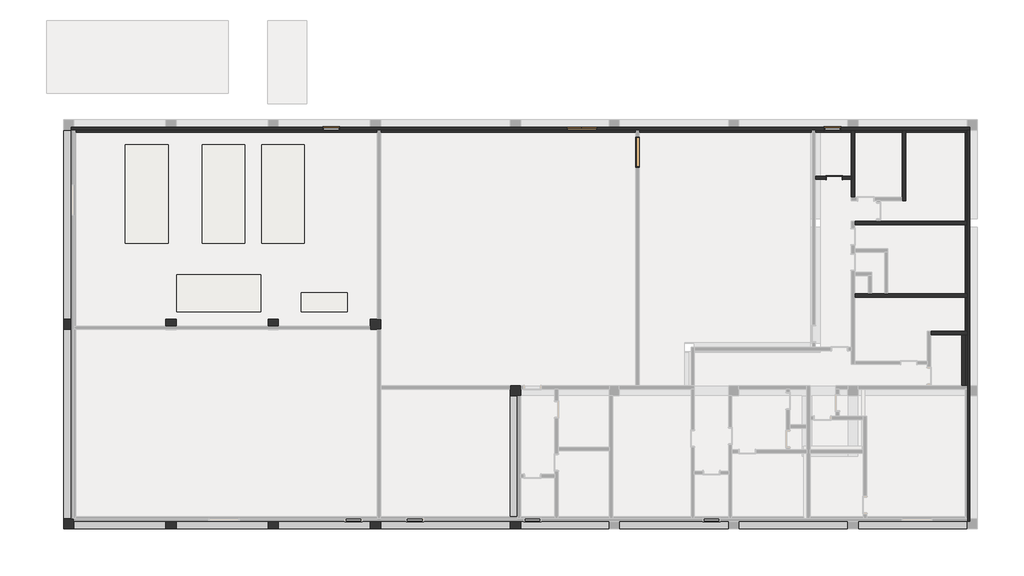
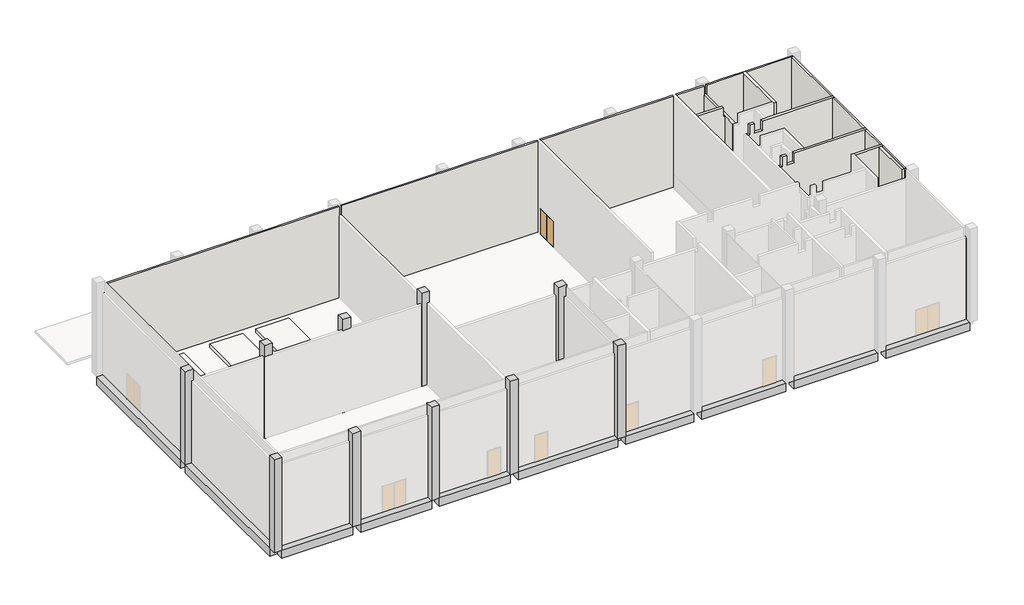
# One storey, part 3 of 4: 19 walls, 10 columns, 5 doors, 5 slabs, 3 beams.
"""IFC4 building model written with IfcOpenShell, lengths in millimetres."""

import ifcopenshell
import ifcopenshell.guid

model = None  # the IFC model being written
_history = None  # IfcOwnerHistory: only IFC2X3 demands one
_inside = {}  # id of a spatial element -> (the spatial element, [elements in it])
_under = {}  # id of a project, library or spatial element -> (it, [spatial elements below it])
_declared = {}  # id of a project -> (the project, [libraries it declares])
_typed = {}  # id of a type object -> (the type object, [elements of that type])
_made_of = {}  # id of a material, layer set ... -> (it, [elements and type objects made of it])


def new_model(schema):
    """Start an empty IFC model of exactly this schema.

    Asked for "IFC4X3", IfcOpenShell would pick the latest addendum, in which some entities
    have other attributes; the version numbers below select the first issue.
    IFC2X3 requires an IfcOwnerHistory on every rooted entity: one is made here for all.
    """
    global model, _history
    if schema == "IFC4X3":
        model = ifcopenshell.file(schema_version=(4, 3, 0, 0))
    else:
        model = ifcopenshell.file(schema=schema)
    _inside.clear()
    _under.clear()
    _declared.clear()
    _typed.clear()
    _made_of.clear()
    _history = None
    if model.schema == "IFC2X3":
        org = make("IfcOrganization", Name="unknown")
        user = make(
            "IfcPersonAndOrganization",
            ThePerson=make("IfcPerson", FamilyName="unknown"),
            TheOrganization=org,
        )
        app = make(
            "IfcApplication",
            ApplicationDeveloper=org,
            Version="unknown",
            ApplicationFullName="unknown",
            ApplicationIdentifier="unknown",
        )
        _history = make(
            "IfcOwnerHistory",
            OwningUser=user,
            OwningApplication=app,
            ChangeAction="ADDED",
            CreationDate=0,
        )
    return model


def make(cls, **values):
    """One entity of the class cls with the attributes given. An attribute that is None is left unset."""
    return model.create_entity(
        cls, **{name: value for name, value in values.items() if value is not None}
    )


def rooted(cls, **values):
    """An entity with a GlobalId (a new one), such as an element, a storey or a relation."""
    return make(cls, GlobalId=ifcopenshell.guid.new(), OwnerHistory=_history, **values)


def si_unit(unit_type, name, prefix=None):
    """IfcSIUnit, for example si_unit("LENGTHUNIT", "METRE", prefix="MILLI")."""
    return make("IfcSIUnit", UnitType=unit_type, Prefix=prefix, Name=name)


def assignment(units):
    """IfcUnitAssignment: the units of a project."""
    return None if units is None else make("IfcUnitAssignment", Units=units)


def point(xyz):
    """IfcCartesianPoint."""
    return None if xyz is None else make("IfcCartesianPoint", Coordinates=xyz)


def direction(xyz):
    """IfcDirection."""
    return None if xyz is None else make("IfcDirection", DirectionRatios=xyz)


def frame(location, z_axis=None, x_axis=None):
    """IfcAxis2Placement3D, a coordinate frame: its origin and axes. An axis left out is left unset."""
    return make(
        "IfcAxis2Placement3D",
        Location=point(location),
        Axis=direction(z_axis),
        RefDirection=direction(x_axis),
    )


def origin():
    """The frame at (0, 0, 0) with its axes left unset."""
    return frame((0.0, 0.0, 0.0))


def origin_with_axes():
    """The frame at (0, 0, 0) with the z axis (0, 0, 1) and the x axis (1, 0, 0) written out."""
    return frame((0.0, 0.0, 0.0), z_axis=(0.0, 0.0, 1.0), x_axis=(1.0, 0.0, 0.0))


def place(relative_to, where):
    """IfcLocalPlacement: puts the frame where relative to a parent placement (None: the world)."""
    return make(
        "IfcLocalPlacement", PlacementRelTo=relative_to, RelativePlacement=where
    )


def context(
    kind, dimensions, precision=None, world=None, true_north=None, identifier=None
):
    """IfcGeometricRepresentationContext, for example the 3D "Model" context."""
    return make(
        "IfcGeometricRepresentationContext",
        ContextIdentifier=identifier,
        ContextType=kind,
        CoordinateSpaceDimension=dimensions,
        Precision=precision,
        WorldCoordinateSystem=world,
        TrueNorth=true_north,
    )


def project(units=None, contexts=None):
    """IfcProject with its units and contexts."""
    return rooted(
        "IfcProject",
        Name="project",
        RepresentationContexts=contexts,
        UnitsInContext=assignment(units),
    )


def spatial(cls, under=None, at=None, **own):
    """A site, building, storey or space (cls), placed at a placement, below another one or the project."""
    s = rooted(cls, ObjectPlacement=at, **own)
    if under is not None:
        _under.setdefault(under.id(), (under, []))[1].append(s)
    return s


def polyline(points):
    """IfcPolyline through the points."""
    return make("IfcPolyline", Points=[point(p) for p in points])


def outline(outer, holes=None, kind="AREA"):
    """IfcArbitraryClosedProfileDef: a profile drawn as a closed curve; with holes, ...WithVoids."""
    if holes is None:
        return make("IfcArbitraryClosedProfileDef", ProfileType=kind, OuterCurve=outer)
    return make(
        "IfcArbitraryProfileDefWithVoids",
        ProfileType=kind,
        OuterCurve=outer,
        InnerCurves=holes,
    )


def extrude(swept, where, along, depth):
    """IfcExtrudedAreaSolid: the profile swept, set in the frame where, extruded along a direction by depth."""
    return make(
        "IfcExtrudedAreaSolid",
        SweptArea=swept,
        Position=where,
        ExtrudedDirection=direction(along),
        Depth=depth,
    )


def faces_of(points, faces, orient=None, outer=None):
    """IfcFace entities. A face is a list of loops; a loop is a list of indices into points, from 0.

    orient and outer hold one flag for each loop. By default every Orientation is true, the
    first loop of a face is its IfcFaceOuterBound and the others are IfcFaceBound.
    """
    made = []
    for i, loops in enumerate(faces):
        bounds = []
        for j, loop in enumerate(loops):
            is_outer = j == 0 if outer is None else outer[i][j]
            bounds.append(
                make(
                    "IfcFaceOuterBound" if is_outer else "IfcFaceBound",
                    Bound=make("IfcPolyLoop", Polygon=[points[k] for k in loop]),
                    Orientation=True if orient is None else orient[i][j],
                )
            )
        made.append(make("IfcFace", Bounds=bounds))
    return made


def faceted_brep(points, faces, orient=None, outer=None, voids=None):
    """IfcFacetedBrep: a solid bounded by flat faces; with voids (closed shells), ...WithVoids."""
    shared = [point(p) for p in points]
    hull = make("IfcClosedShell", CfsFaces=faces_of(shared, faces, orient, outer))
    if voids is None:
        return make("IfcFacetedBrep", Outer=hull)
    return make(
        "IfcFacetedBrepWithVoids",
        Outer=hull,
        Voids=[
            make(cls, CfsFaces=faces_of(shared, fs, o, b)) for cls, fs, o, b in voids
        ],
    )


def shape(context_of_items, identifier, shape_type, items):
    """IfcShapeRepresentation: the items that make up one representation, for example the "Body"."""
    return make(
        "IfcShapeRepresentation",
        ContextOfItems=context_of_items,
        RepresentationIdentifier=identifier,
        RepresentationType=shape_type,
        Items=items,
    )


def source(mapping_origin, context_of_items, identifier, shape_type, items):
    """IfcRepresentationMap: a shape defined once, which mapped items show again and again."""
    return make(
        "IfcRepresentationMap",
        MappingOrigin=mapping_origin,
        MappedRepresentation=shape(context_of_items, identifier, shape_type, items),
    )


def transform(
    local_origin,
    x_axis=None,
    y_axis=None,
    z_axis=None,
    scale=None,
    scale2=None,
    scale3=None,
    uniform=True,
):
    """IfcCartesianTransformationOperator3D, or its non-uniform kind. x_axis, y_axis, z_axis: its Axis1, 2, 3."""
    if uniform:
        return make(
            "IfcCartesianTransformationOperator3D",
            Axis1=direction(x_axis),
            Axis2=direction(y_axis),
            LocalOrigin=point(local_origin),
            Scale=scale,
            Axis3=direction(z_axis),
        )
    return make(
        "IfcCartesianTransformationOperator3DnonUniform",
        Axis1=direction(x_axis),
        Axis2=direction(y_axis),
        LocalOrigin=point(local_origin),
        Scale=scale,
        Axis3=direction(z_axis),
        Scale2=scale2,
        Scale3=scale3,
    )


def mapped(mapping_source, mapping_target):
    """IfcMappedItem: shows the shape of a source again, moved by a transform."""
    return make(
        "IfcMappedItem", MappingSource=mapping_source, MappingTarget=mapping_target
    )


def made_of(thing, what):
    """Note that an element or type object is made of a material, layer set ...; save() writes the relation."""
    if what is not None:
        _made_of.setdefault(what.id(), (what, []))[1].append(thing)
    return thing


def element(
    cls,
    number,
    at=None,
    inside=None,
    cuts=None,
    type_object=None,
    material=None,
    context=None,
    identifier="Body",
    shape_type=None,
    held_by="IfcProductDefinitionShape",
    body=None,
    shapes=None,
    **own,
):
    """One element of the class cls, such as IfcWall. Its Tag is "e" and its number.

    at: its placement. inside: the storey or other place that contains it. cuts: it is an
    opening in that element (IfcRelVoidsElement). A single representation is given by context,
    identifier, shape_type and body (its items); several are given by shapes. held_by: the class
    of the entity that holds the representations. save() writes the other relations.
    """
    e = rooted(cls, Tag="e%d" % number, ObjectPlacement=at, **own)
    if body is not None:
        shapes = [shape(context, identifier, shape_type, body)]
    if shapes is not None:
        e.Representation = make(held_by, Representations=shapes)
    if inside is not None:
        _inside.setdefault(inside.id(), (inside, []))[1].append(e)
    if cuts is not None:
        rooted(
            "IfcRelVoidsElement", RelatingBuildingElement=cuts, RelatedOpeningElement=e
        )
    if type_object is not None:
        _typed.setdefault(type_object.id(), (type_object, []))[1].append(e)
    return made_of(e, material)


def aggregate(whole, parts):
    """IfcRelAggregates: a whole, such as a stair, and the parts it consists of."""
    return rooted("IfcRelAggregates", RelatingObject=whole, RelatedObjects=parts)


def save(model, path):
    """Write the relations noted so far, then the file.

    IfcRelAggregates (storeys below a building ...), IfcRelContainedInSpatialStructure (elements
    in a storey), IfcRelDefinesByType, IfcRelAssociatesMaterial and IfcRelDeclares: one each for
    every whole, place, type object, material and project.
    """
    for whole, parts in _under.values():
        aggregate(whole, parts)
    for where, things in _inside.values():
        rooted(
            "IfcRelContainedInSpatialStructure",
            RelatedElements=things,
            RelatingStructure=where,
        )
    for kind, things in _typed.values():
        rooted("IfcRelDefinesByType", RelatedObjects=things, RelatingType=kind)
    for what, things in _made_of.values():
        rooted("IfcRelAssociatesMaterial", RelatedObjects=things, RelatingMaterial=what)
    for by, libraries in _declared.values():
        rooted("IfcRelDeclares", RelatingContext=by, RelatedDefinitions=libraries)
    model.write(path)


def double_door_steel_580823b0(model_context):
    return source(origin(), model_context, "Body", "SolidModel", [
        extrude(outline(polyline([(880.0, 35.0), (0.0, 35.0), (0.0, 75.0), (880.0, 75.0), (880.0, 35.0)])), frame((0.0, 0.0, 20.0), z_axis=(0.0, 0.0, 1.0), x_axis=(1.0, 0.0, 0.0)), (0.0, 0.0, 1.0), 2060.0),
        extrude(outline(polyline([(0.0, 35.0), (-880.0, 35.0), (-880.0, 75.0), (0.0, 75.0), (0.0, 35.0)])), frame((0.0, 0.0, 20.0), z_axis=(0.0, 0.0, 1.0), x_axis=(1.0, 0.0, 0.0)), (0.0, 0.0, 1.0), 2060.0),
        faceted_brep([(900.0, -75.0, 2100.0), (900.0, 75.0, 2100.0), (-900.0, 75.0, 2100.0), (-900.0, -75.0, 2100.0), (865.0, 35.0, 2065.0), (865.0, -75.0, 2065.0), (-865.0, -75.0, 2065.0), (-865.0, 35.0, 2065.0), (880.0, 75.0, 2080.0), (880.0, 35.0, 2080.0), (-880.0, 35.0, 2080.0), (-880.0, 75.0, 2080.0), (-900.0, 75.0, 0.0), (-900.0, -75.0, 0.0), (-865.0, -75.0, 35.0), (-865.0, 35.0, 35.0), (-880.0, 35.0, 20.0), (-880.0, 75.0, 20.0), (900.0, 75.0, 0.0), (880.0, 75.0, 20.0), (900.0, -75.0, 0.0), (865.0, -75.0, 35.0), (865.0, 35.0, 35.0), (880.0, 35.0, 20.0)], [[[0, 1, 2, 3]], [[4, 5, 6, 7]], [[8, 9, 10, 11]], [[3, 2, 12, 13]], [[7, 6, 14, 15]], [[11, 10, 16, 17]], [[18, 12, 2, 1], [8, 11, 17, 19]], [[13, 12, 18, 20]], [[0, 3, 13, 20], [21, 14, 6, 5]], [[15, 14, 21, 22]], [[23, 16, 10, 9], [4, 7, 15, 22]], [[17, 16, 23, 19]], [[20, 18, 1, 0]], [[22, 21, 5, 4]], [[19, 23, 9, 8]]]),
    ])


def double_door_steel_63a69c0a(model_context):
    return source(origin(), model_context, "Body", "SolidModel", [
        extrude(outline(polyline([(880.0, -60.0), (880.0, -100.0), (0.0, -100.0), (0.0, -60.0), (880.0, -60.0)])), frame((0.0, 0.0, 20.0), z_axis=(0.0, 0.0, 1.0), x_axis=(1.0, 0.0, 0.0)), (0.0, 0.0, 1.0), 2060.0),
        extrude(outline(polyline([(0.0, -60.0), (0.0, -100.0), (-880.0, -100.0), (-880.0, -60.0), (0.0, -60.0)])), frame((0.0, 0.0, 20.0), z_axis=(0.0, 0.0, 1.0), x_axis=(1.0, 0.0, 0.0)), (0.0, 0.0, 1.0), 2060.0),
        faceted_brep([(900.0, 100.0, 2100.0), (-900.0, 100.0, 2100.0), (-900.0, -100.0, 2100.0), (900.0, -100.0, 2100.0), (865.0, -60.0, 2065.0), (-865.0, -60.0, 2065.0), (-865.0, 100.0, 2065.0), (865.0, 100.0, 2065.0), (880.0, -100.0, 2080.0), (-880.0, -100.0, 2080.0), (-880.0, -60.0, 2080.0), (880.0, -60.0, 2080.0), (-900.0, 100.0, 0.0), (-900.0, -100.0, 0.0), (-865.0, -60.0, 35.0), (-865.0, 100.0, 35.0), (-880.0, -100.0, 20.0), (-880.0, -60.0, 20.0), (900.0, -100.0, 0.0), (880.0, -100.0, 20.0), (900.0, 100.0, 0.0), (865.0, 100.0, 35.0), (865.0, -60.0, 35.0), (880.0, -60.0, 20.0)], [[[0, 1, 2, 3]], [[4, 5, 6, 7]], [[8, 9, 10, 11]], [[1, 12, 13, 2]], [[5, 14, 15, 6]], [[9, 16, 17, 10]], [[18, 3, 2, 13], [8, 19, 16, 9]], [[12, 20, 18, 13]], [[0, 20, 12, 1], [21, 7, 6, 15]], [[14, 22, 21, 15]], [[23, 11, 10, 17], [4, 22, 14, 5]], [[16, 19, 23, 17]], [[20, 0, 3, 18]], [[22, 4, 7, 21]], [[19, 8, 11, 23]]]),
    ])


def single_door_steel_b319cbd1(model_context):
    return source(origin(), model_context, "Body", "SolidModel", [
        extrude(outline(polyline([(480.0, -105.0), (-480.0, -105.0), (-480.0, -70.0), (480.0, -70.0), (480.0, -105.0)])), origin_with_axes(), (0.0, 0.0, 1.0), 2130.0),
        faceted_brep([(480.0, -105.0, 0.0), (480.0, -70.0, 0.0), (460.0, -70.0, 0.0), (460.0, 70.0, 0.0), (480.0, 70.0, 0.0), (480.0, 105.0, 0.0), (510.0, 105.0, 0.0), (510.0, -105.0, 0.0), (510.0, -105.0, 2160.0), (-510.0, -105.0, 2160.0), (-510.0, -105.0, 0.0), (-480.0, -105.0, 0.0), (-480.0, -105.0, 2130.0), (480.0, -105.0, 2130.0), (510.0, 105.0, 2160.0), (480.0, 105.0, 2130.0), (-480.0, 105.0, 2130.0), (-480.0, 105.0, 0.0), (-510.0, 105.0, 0.0), (-510.0, 105.0, 2160.0), (480.0, 70.0, 2130.0), (460.0, 70.0, 2110.0), (-460.0, 70.0, 2110.0), (-460.0, 70.0, 0.0), (-480.0, 70.0, 0.0), (-480.0, 70.0, 2130.0), (460.0, -70.0, 2110.0), (480.0, -70.0, 2130.0), (-480.0, -70.0, 2130.0), (-480.0, -70.0, 0.0), (-460.0, -70.0, 0.0), (-460.0, -70.0, 2110.0)], [[[0, 1, 2, 3, 4, 5, 6, 7]], [[7, 8, 9, 10, 11, 12, 13, 0]], [[6, 14, 8, 7]], [[5, 15, 16, 17, 18, 19, 14, 6]], [[4, 20, 15, 5]], [[3, 21, 22, 23, 24, 25, 20, 4]], [[2, 26, 21, 3]], [[1, 27, 28, 29, 30, 31, 26, 2]], [[0, 13, 27, 1]], [[12, 11, 29, 28]], [[11, 10, 18, 17, 24, 23, 30, 29]], [[19, 18, 10, 9]], [[25, 24, 17, 16]], [[31, 30, 23, 22]], [[14, 19, 9, 8]], [[20, 25, 16, 15]], [[26, 31, 22, 21]], [[13, 12, 28, 27]]]),
    ])


def single_door_steel_f73fbc53(model_context):
    return source(origin(), model_context, "Body", "SolidModel", [
        extrude(outline(polyline([(480.0, -130.0), (-480.0, -130.0), (-480.0, -95.0), (480.0, -95.0), (480.0, -130.0)])), origin_with_axes(), (0.0, 0.0, 1.0), 2130.0),
        faceted_brep([(480.0, -130.0, 0.0), (480.0, -95.0, 0.0), (460.0, -95.0, 0.0), (460.0, 95.0, 0.0), (480.0, 95.0, 0.0), (480.0, 130.0, 0.0), (510.0, 130.0, 0.0), (510.0, -130.0, 0.0), (510.0, -130.0, 2160.0), (-510.0, -130.0, 2160.0), (-510.0, -130.0, 0.0), (-480.0, -130.0, 0.0), (-480.0, -130.0, 2130.0), (480.0, -130.0, 2130.0), (510.0, 130.0, 2160.0), (480.0, 130.0, 2130.0), (-480.0, 130.0, 2130.0), (-480.0, 130.0, 0.0), (-510.0, 130.0, 0.0), (-510.0, 130.0, 2160.0), (480.0, 95.0, 2130.0), (460.0, 95.0, 2110.0), (-460.0, 95.0, 2110.0), (-460.0, 95.0, 0.0), (-480.0, 95.0, 0.0), (-480.0, 95.0, 2130.0), (460.0, -95.0, 2110.0), (480.0, -95.0, 2130.0), (-480.0, -95.0, 2130.0), (-480.0, -95.0, 0.0), (-460.0, -95.0, 0.0), (-460.0, -95.0, 2110.0)], [[[0, 1, 2, 3, 4, 5, 6, 7]], [[7, 8, 9, 10, 11, 12, 13, 0]], [[6, 14, 8, 7]], [[5, 15, 16, 17, 18, 19, 14, 6]], [[4, 20, 15, 5]], [[3, 21, 22, 23, 24, 25, 20, 4]], [[2, 26, 21, 3]], [[1, 27, 28, 29, 30, 31, 26, 2]], [[0, 13, 27, 1]], [[12, 11, 29, 28]], [[11, 10, 18, 17, 24, 23, 30, 29]], [[19, 18, 10, 9]], [[25, 24, 17, 16]], [[31, 30, 23, 22]], [[14, 19, 9, 8]], [[20, 25, 16, 15]], [[26, 31, 22, 21]], [[13, 12, 28, 27]]]),
    ])


model = new_model("IFC4")

# Units and contexts
model_context = context("Model", 3, world=origin())
ifc_project = project(units=[si_unit("LENGTHUNIT", "METRE", prefix="MILLI")], contexts=[model_context])

# Site, building, storey
site = spatial("IfcSite", under=ifc_project)
building = spatial("IfcBuilding", under=site)
storey = spatial("IfcBuildingStorey", under=building, Name="TOC(GF)", Elevation=97049.9618634)

# Beams
placement = place(None, origin())
element("IfcBeam", 1, ObjectType="RC Beam_Rectangular : H_SB_AR S16_TG-UG_TG1 600x650", at=placement, inside=storey, context=model_context, shape_type="Brep", body=[
    faceted_brep([(300.0, -19200.0, 97049.9618634), (300.0, -19800.0, 97049.9618634), (5700.0, -19800.0, 97049.9618634), (5700.0, -19200.0, 97049.9618634), (300.0, -19200.0, 96399.9618634), (300.0, -19200.0, 96849.9618634), (5700.0, -19200.0, 96399.9618634), (300.0, -19800.0, 96399.9618634), (5700.0, -19800.0, 96399.9618634)], [[[0, 1, 2, 3]], [[4, 5, 0, 3, 6]], [[7, 4, 6, 8]], [[1, 7, 8, 2]], [[1, 0, 5, 4, 7]], [[3, 2, 8, 6]]]),
    faceted_brep([(26500.0, -19800.0, 97049.9618634), (26500.0, -19200.0, 97049.9618634), (26500.0, -19200.0, 96849.9618634), (26500.0, -19200.0, 96399.9618634), (26500.0, -19800.0, 96399.9618634), (31700.0, -19200.0, 97049.9618634), (31700.0, -19800.0, 97049.9618634), (31700.0, -19800.0, 96399.9618634), (31700.0, -19200.0, 96399.9618634)], [[[0, 1, 2, 3, 4]], [[5, 6, 7, 8]], [[1, 0, 6, 5]], [[3, 2, 1, 5, 8]], [[4, 3, 8, 7]], [[0, 4, 7, 6]]]),
    faceted_brep([(25900.0, -19200.0, 97049.9618634), (25900.0, -19800.0, 97049.9618634), (25900.0, -19800.0, 96399.9618634), (25900.0, -19200.0, 96399.9618634), (25900.0, -19200.0, 96849.9618634), (18300.0, -19800.0, 97049.9618634), (18300.0, -19200.0, 97049.9618634), (18300.0, -19200.0, 96399.9618634), (18300.0, -19800.0, 96399.9618634)], [[[0, 1, 2, 3, 4]], [[5, 6, 7, 8]], [[1, 0, 6, 5]], [[0, 4, 3, 7, 6]], [[3, 2, 8, 7]], [[2, 1, 5, 8]]]),
    faceted_brep([(32300.0, -19800.0, 97049.9618634), (32300.0, -19200.0, 97049.9618634), (32300.0, -19200.0, 96399.9618634), (32300.0, -19800.0, 96399.9618634), (38700.0, -19200.0, 97049.9618634), (38700.0, -19800.0, 97049.9618634), (38700.0, -19800.0, 96399.9618634), (38700.0, -19200.0, 96399.9618634)], [[[0, 1, 2, 3]], [[4, 5, 6, 7]], [[1, 0, 5, 4]], [[2, 1, 4, 7]], [[3, 2, 7, 6]], [[0, 3, 6, 5]]]),
    faceted_brep([(39300.0, -19800.0, 97049.9618634), (39300.0, -19200.0, 97049.9618634), (39300.0, -19200.0, 96399.9618634), (39300.0, -19800.0, 96399.9618634), (45700.0, -19200.0, 97049.9618634), (45700.0, -19800.0, 97049.9618634), (45700.0, -19800.0, 96399.9618634), (45700.0, -19200.0, 96399.9618634)], [[[0, 1, 2, 3]], [[4, 5, 6, 7]], [[1, 0, 5, 4]], [[2, 1, 4, 7]], [[3, 2, 7, 6]], [[0, 3, 6, 5]]]),
    faceted_brep([(46300.0, -19800.0, 97049.9618634), (46300.0, -19200.0, 97049.9618634), (46300.0, -19200.0, 96399.9618634), (46300.0, -19800.0, 96399.9618634), (52700.0, -19200.0, 97049.9618634), (52700.0, -19800.0, 97049.9618634), (52700.0, -19800.0, 96399.9618634), (52700.0, -19200.0, 96399.9618634), (52700.0, -19200.0, 96849.9618634)], [[[0, 1, 2, 3]], [[4, 5, 6, 7, 8]], [[1, 0, 5, 4]], [[2, 1, 4, 8, 7]], [[3, 2, 7, 6]], [[0, 3, 6, 5]]]),
    faceted_brep([(6300.0, -19800.0, 97049.9618634), (6300.0, -19200.0, 97049.9618634), (6300.0, -19200.0, 96399.9618634), (6300.0, -19800.0, 96399.9618634), (11700.0, -19200.0, 97049.9618634), (11700.0, -19800.0, 97049.9618634), (11700.0, -19800.0, 96399.9618634), (11700.0, -19200.0, 96399.9618634)], [[[0, 1, 2, 3]], [[4, 5, 6, 7]], [[1, 0, 5, 4]], [[2, 1, 4, 7]], [[3, 2, 7, 6]], [[0, 3, 6, 5]]]),
    faceted_brep([(12300.0, -19800.0, 97049.9618634), (12300.0, -19200.0, 97049.9618634), (12300.0, -19200.0, 96399.9618634), (12300.0, -19800.0, 96399.9618634), (17700.0, -19200.0, 97049.9618634), (17700.0, -19800.0, 97049.9618634), (17700.0, -19800.0, 96399.9618634), (17700.0, -19200.0, 96399.9618634)], [[[0, 1, 2, 3]], [[4, 5, 6, 7]], [[1, 0, 5, 4]], [[2, 1, 4, 7]], [[3, 2, 7, 6]], [[0, 3, 6, 5]]]),
])
element("IfcBeam", 2, ObjectType="RC Beam_Rectangular : H_SB_AR S16_TG-UG_TG1 600x650", at=placement, inside=storey, context=model_context, shape_type="Brep", body=[
    faceted_brep([(300.0, 3600.0, 97049.9618634), (-300.0, 3600.0, 97049.9618634), (-300.0, -7500.0, 97049.9618634), (300.0, -7500.0, 97049.9618634), (300.0, 3600.0, 96399.9618634), (300.0, 3600.0, 96849.9618634), (300.0, -7500.0, 96399.9618634), (-300.0, 3600.0, 96399.9618634), (-300.0, -7500.0, 96399.9618634)], [[[0, 1, 2, 3]], [[4, 5, 0, 3, 6]], [[7, 4, 6, 8]], [[8, 2, 1, 7]], [[0, 5, 4, 7, 1]], [[3, 2, 8, 6]]]),
    faceted_brep([(300.0, -19200.0, 96399.9618634), (300.0, -19200.0, 96849.9618634), (300.0, -19200.0, 97049.9618634), (-300.0, -19200.0, 97049.9618634), (-300.0, -19200.0, 96399.9618634), (-300.0, -8100.0, 97049.9618634), (300.0, -8100.0, 97049.9618634), (300.0, -8100.0, 96399.9618634), (-300.0, -8100.0, 96399.9618634)], [[[0, 1, 2, 3, 4]], [[5, 6, 7, 8]], [[3, 2, 6, 5]], [[2, 1, 0, 7, 6]], [[0, 4, 8, 7]], [[4, 3, 5, 8]]]),
])
element("IfcBeam", 3, ObjectType="RC Beam_Rectangular : H_SB_AR S16_TG-UG_TG1 600x650", at=placement, inside=storey, context=model_context, shape_type="Brep", body=[
    faceted_brep([(26500.0, -12000.0, 97049.9618634), (25900.0, -12000.0, 97049.9618634), (25900.0, -19200.0, 97049.9618634), (26500.0, -19200.0, 97049.9618634), (25900.0, -12000.0, 96399.9618634), (25900.0, -19200.0, 96399.9618634), (25900.0, -19200.0, 96849.9618634), (26500.0, -12000.0, 96399.9618634), (26500.0, -19200.0, 96399.9618634), (26500.0, -12000.0, 96849.9618634), (26500.0, -19200.0, 96849.9618634)], [[[0, 1, 2, 3]], [[1, 4, 5, 6, 2]], [[4, 7, 8, 5]], [[7, 9, 0, 3, 10, 8]], [[0, 9, 7, 4, 1]], [[3, 2, 6, 5, 8, 10]]]),
])

# Columns
element("IfcColumn", 4, ObjectType="RC_Column_Rectangular : H_SC_AR S15_RC Col-AG_C1 600x600", at=placement, inside=storey, context=model_context, shape_type="Brep", body=[
    faceted_brep([(300.0, -19200.0, 97049.9618634), (300.0, -19350.0, 97049.9618634), (300.0, -19800.0, 97049.9618634), (-300.0, -19800.0, 97049.9618634), (-300.0, -19200.0, 97049.9618634), (300.0, -19200.0, 104550.0), (300.0, -19800.0, 104550.0), (300.0, -19200.0, 103650.0), (-300.0, -19800.0, 104550.0), (-300.0, -19200.0, 104550.0)], [[[0, 1, 2, 3, 4]], [[5, 6, 2, 1, 0, 7]], [[6, 8, 3, 2]], [[8, 9, 4, 3]], [[9, 5, 7, 0, 4]], [[5, 9, 8, 6]]]),
])
element("IfcColumn", 5, ObjectType="RC_Column_Rectangular : H_SC_AR S15_RC Col-AG_C1 600x600", at=placement, inside=storey, context=model_context, shape_type="Brep", body=[
    faceted_brep([(300.0, -7500.0, 97049.9618634), (300.0, -8100.0, 97049.9618634), (-300.0, -8100.0, 97049.9618634), (-300.0, -7500.0, 97049.9618634), (300.0, -7500.0, 104550.0), (300.0, -8100.0, 104550.0), (300.0, -8100.0, 103650.0), (300.0, -7500.0, 103650.0), (-300.0, -8100.0, 104550.0), (-300.0, -8100.0, 103650.0), (-300.0, -7500.0, 104550.0), (-300.0, -7500.0, 103650.0)], [[[0, 1, 2, 3]], [[4, 5, 6, 1, 0, 7]], [[5, 8, 9, 2, 1, 6]], [[8, 10, 11, 3, 2, 9]], [[10, 4, 7, 0, 3, 11]], [[4, 10, 8, 5]]]),
])
element("IfcColumn", 6, ObjectType="RC_Column_Rectangular : H_SC_AR S15_RC Col-AG_C1 600x600", at=placement, inside=storey, context=model_context, shape_type="Brep", body=[
    faceted_brep([(26500.0, -19200.0, 97049.9618634), (26500.0, -19800.0, 97049.9618634), (25900.0, -19800.0, 97049.9618634), (25900.0, -19200.0, 97049.9618634), (26500.0, -19200.0, 104550.0), (26500.0, -19800.0, 104550.0), (26500.0, -19800.0, 103650.0), (26500.0, -19200.0, 103650.0), (25900.0, -19800.0, 104550.0), (25900.0, -19800.0, 103650.0), (25900.0, -19200.0, 104550.0), (25900.0, -19200.0, 103650.0), (25950.0, -19200.0, 104550.0), (26450.0, -19200.0, 104550.0)], [[[0, 1, 2, 3]], [[4, 5, 6, 1, 0, 7]], [[5, 8, 9, 2, 1, 6]], [[8, 10, 11, 3, 2, 9]], [[10, 12, 13, 4, 7, 0, 3, 11]], [[4, 13, 12, 10, 8, 5]]]),
])
element("IfcColumn", 7, ObjectType="RC_Column_Rectangular : H_SC_AR S15_RC Col-AG_C1 600x600", at=placement, inside=storey, context=model_context, shape_type="Brep", body=[
    faceted_brep([(6300.0, -19200.0, 97049.9618634), (6300.0, -19800.0, 97049.9618634), (5700.0, -19800.0, 97049.9618634), (5700.0, -19200.0, 97049.9618634), (6300.0, -19200.0, 104550.0), (6300.0, -19800.0, 104550.0), (6300.0, -19800.0, 103650.0), (6300.0, -19200.0, 103650.0), (5700.0, -19800.0, 104550.0), (5700.0, -19800.0, 103650.0), (5700.0, -19200.0, 104550.0), (5700.0, -19200.0, 103650.0), (5800.0, -19200.0, 104550.0), (6200.0, -19200.0, 104550.0)], [[[0, 1, 2, 3]], [[4, 5, 6, 1, 0, 7]], [[5, 8, 9, 2, 1, 6]], [[8, 10, 11, 3, 2, 9]], [[10, 12, 13, 4, 7, 0, 3, 11]], [[4, 13, 12, 10, 8, 5]]]),
])
element("IfcColumn", 8, ObjectType="RC_Column_Rectangular : H_SC_AR S15_RC Col-AG_C1 600x600", at=placement, inside=storey, context=model_context, shape_type="Brep", body=[
    faceted_brep([(6300.0, -7500.0, 97049.9618634), (6300.0, -8100.0, 97049.9618634), (5700.0, -8100.0, 97049.9618634), (5700.0, -7500.0, 97049.9618634), (6300.0, -7500.0, 104550.0), (6300.0, -8100.0, 104550.0), (6300.0, -8100.0, 103650.0), (6300.0, -7500.0, 103650.0), (6200.0, -8100.0, 104550.0), (5800.0, -8100.0, 104550.0), (5700.0, -8100.0, 104550.0), (5700.0, -8100.0, 103650.0), (5700.0, -7500.0, 104550.0), (5700.0, -7500.0, 103650.0), (5800.0, -7500.0, 104550.0), (6200.0, -7500.0, 104550.0)], [[[0, 1, 2, 3]], [[4, 5, 6, 1, 0, 7]], [[5, 8, 9, 10, 11, 2, 1, 6]], [[10, 12, 13, 3, 2, 11]], [[12, 14, 15, 4, 7, 0, 3, 13]], [[4, 15, 14, 12, 10, 9, 8, 5]]]),
])
element("IfcColumn", 9, ObjectType="RC_Column_Rectangular : H_SC_AR S15_RC Col-AG_C1 600x600", at=placement, inside=storey, context=model_context, shape_type="Brep", body=[
    faceted_brep([(12300.0, -19200.0, 97049.9618634), (12300.0, -19800.0, 97049.9618634), (11700.0, -19800.0, 97049.9618634), (11700.0, -19200.0, 97049.9618634), (12300.0, -19200.0, 104550.0), (12300.0, -19800.0, 104550.0), (12300.0, -19800.0, 103650.0), (12300.0, -19200.0, 103650.0), (11700.0, -19800.0, 104550.0), (11700.0, -19800.0, 103650.0), (11700.0, -19200.0, 104550.0), (11700.0, -19200.0, 103650.0), (11800.0, -19200.0, 104550.0), (12200.0, -19200.0, 104550.0)], [[[0, 1, 2, 3]], [[4, 5, 6, 1, 0, 7]], [[5, 8, 9, 2, 1, 6]], [[8, 10, 11, 3, 2, 9]], [[10, 12, 13, 4, 7, 0, 3, 11]], [[4, 13, 12, 10, 8, 5]]]),
])
element("IfcColumn", 10, ObjectType="RC_Column_Rectangular : H_SC_AR S15_RC Col-AG_C1 600x600", at=placement, inside=storey, context=model_context, shape_type="Brep", body=[
    faceted_brep([(12300.0, -7500.0, 97049.9618634), (12300.0, -8100.0, 97049.9618634), (11700.0, -8100.0, 97049.9618634), (11700.0, -7500.0, 97049.9618634), (12300.0, -7500.0, 104550.0), (12300.0, -8100.0, 104550.0), (12300.0, -8100.0, 103650.0), (12300.0, -7500.0, 103650.0), (12200.0, -8100.0, 104550.0), (11800.0, -8100.0, 104550.0), (11700.0, -8100.0, 104550.0), (11700.0, -8100.0, 103650.0), (11700.0, -7500.0, 104550.0), (11700.0, -7500.0, 103650.0), (11800.0, -7500.0, 104550.0), (12200.0, -7500.0, 104550.0)], [[[0, 1, 2, 3]], [[4, 5, 6, 1, 0, 7]], [[5, 8, 9, 10, 11, 2, 1, 6]], [[10, 12, 13, 3, 2, 11]], [[12, 14, 15, 4, 7, 0, 3, 13]], [[4, 15, 14, 12, 10, 9, 8, 5]]]),
])
element("IfcColumn", 11, ObjectType="RC_Column_Rectangular : H_SC_AR S15_RC Col-AG_C1 600x600", at=placement, inside=storey, context=model_context, shape_type="Brep", body=[
    faceted_brep([(18300.0, -19200.0, 97049.9618634), (18300.0, -19800.0, 97049.9618634), (17700.0, -19800.0, 97049.9618634), (17700.0, -19200.0, 97049.9618634), (18300.0, -19200.0, 104550.0), (18300.0, -19800.0, 104550.0), (18300.0, -19800.0, 103650.0), (18300.0, -19200.0, 103650.0), (17700.0, -19800.0, 104550.0), (17700.0, -19800.0, 103650.0), (17700.0, -19200.0, 104550.0), (17700.0, -19200.0, 103650.0)], [[[0, 1, 2, 3]], [[4, 5, 6, 1, 0, 7]], [[5, 8, 9, 2, 1, 6]], [[8, 10, 11, 3, 2, 9]], [[10, 4, 7, 0, 3, 11]], [[4, 10, 8, 5]]]),
])
element("IfcColumn", 12, ObjectType="RC_Column_Rectangular : H_SC_AR S15_RC Col-AG_C1 600x600", at=placement, inside=storey, context=model_context, shape_type="Brep", body=[
    faceted_brep([(18300.0, -7500.0, 97049.9618634), (18300.0, -8100.0, 97049.9618634), (17700.0, -8100.0, 97049.9618634), (17700.0, -7500.0, 97049.9618634), (18300.0, -7500.0, 104550.0), (18300.0, -8100.0, 104550.0), (18300.0, -8100.0, 103650.0), (18300.0, -7500.0, 103650.0), (17700.0, -8100.0, 104550.0), (17700.0, -8100.0, 103650.0), (17700.0, -7500.0, 104550.0), (17700.0, -7500.0, 103650.0)], [[[0, 1, 2, 3]], [[4, 5, 6, 1, 0, 7]], [[5, 8, 9, 2, 1, 6]], [[8, 10, 11, 3, 2, 9]], [[10, 4, 7, 0, 3, 11]], [[4, 10, 8, 5]]]),
])
element("IfcColumn", 13, ObjectType="RC_Column_Rectangular : H_SC_AR S15_RC Col-AG_C2 600x600 2", at=placement, inside=storey, context=model_context, shape_type="SweptSolid", body=[
    extrude(outline(polyline([(26500.0, -11400.0), (26500.0, -12000.0), (25900.0, -12000.0), (25900.0, -11400.0), (26500.0, -11400.0)])), frame((0.0, 0.0, 97049.9618634), z_axis=(0.0, 0.0, 1.0), x_axis=(1.0, 0.0, 0.0)), (0.0, 0.0, 1.0), 7500.0381366),
])

# Doors
double_door_steel_shape = double_door_steel_580823b0(model_context)
element("IfcDoor", 14, ObjectType="Double Door_Steel : H_DR_AR B12_Door_Double FSD 02", at=placement, inside=storey, context=model_context, shape_type="MappedRepresentation", body=[
    mapped(double_door_steel_shape, transform((30100.0, 3675.0, 97049.9618634), x_axis=(1.0, 0.0, 0.0), y_axis=(0.0, 1.0, 0.0), z_axis=(0.0, 0.0, 1.0))),
])
double_door_steel_2_shape = double_door_steel_63a69c0a(model_context)
element("IfcDoor", 15, ObjectType="Double Door_Steel : H_DR_AR B12_Door_Double FSD 02", at=placement, inside=storey, context=model_context, shape_type="MappedRepresentation", body=[
    mapped(double_door_steel_2_shape, transform((33350.0, 2300.0, 97049.9618634), x_axis=(0.0, -1.0, 0.0), y_axis=(1.0, 0.0, 0.0), z_axis=(0.0, 0.0, 1.0))),
])
single_door_steel_shape = single_door_steel_b319cbd1(model_context)
element("IfcDoor", 16, ObjectType="Single Door_Steel : H_DR_AR B12_Door_Single FSD 01", at=placement, inside=storey, context=model_context, shape_type="MappedRepresentation", body=[
    mapped(single_door_steel_shape, transform((44800.0, 3675.0, 97049.9618634), x_axis=(-1.0, 0.0, 0.0), y_axis=(0.0, -1.0, 0.0), z_axis=(0.0, 0.0, 1.0))),
])
element("IfcDoor", 17, ObjectType="Single Door_Steel : H_DR_AR B12_Door_Single FSD 01", at=placement, inside=storey, context=model_context, shape_type="MappedRepresentation", body=[
    mapped(single_door_steel_shape, transform((15400.0, 3675.0, 97049.9618634), x_axis=(-1.0, 0.0, 0.0), y_axis=(0.0, -1.0, 0.0), z_axis=(0.0, 0.0, 1.0))),
])
single_door_steel_2_shape = single_door_steel_f73fbc53(model_context)
element("IfcDoor", 18, ObjectType="Single Door_Steel : H_DR_AR B12_Door_Single FSD 01", at=placement, inside=storey, context=model_context, shape_type="MappedRepresentation", body=[
    mapped(single_door_steel_2_shape, transform((44900.0, 800.0, 97049.9618634), x_axis=(-1.0, 0.0, 0.0), y_axis=(0.0, -1.0, 0.0), z_axis=(0.0, 0.0, 1.0))),
])

# Slabs
element("IfcSlab", 19, ObjectType="H_SF_AR B01_EQ Fdn_EF3 2500x5800x300", at=placement, inside=storey, context=model_context, shape_type="SweptSolid", body=[
    extrude(outline(polyline([(5825.0, 2750.0), (5825.0, -3050.0), (3325.0, -3050.0), (3325.0, 2750.0), (5825.0, 2750.0)])), frame((0.0, 0.0, 97049.9618634), z_axis=(0.0, 0.0, 1.0), x_axis=(1.0, 0.0, 0.0)), (0.0, 0.0, 1.0), 300.0),
])
element("IfcSlab", 20, ObjectType="H_SF_AR B01_EQ Fdn_EF3 2500x5800x300", at=placement, inside=storey, context=model_context, shape_type="SweptSolid", body=[
    extrude(outline(polyline([(10325.0, 2750.0), (10325.0, -3050.0), (7825.0, -3050.0), (7825.0, 2750.0), (10325.0, 2750.0)])), frame((0.0, 0.0, 97049.9618634), z_axis=(0.0, 0.0, 1.0), x_axis=(1.0, 0.0, 0.0)), (0.0, 0.0, 1.0), 300.0),
])
element("IfcSlab", 21, ObjectType="H_SF_AR B01_EQ Fdn_EF3 2500x5800x300", at=placement, inside=storey, context=model_context, shape_type="SweptSolid", body=[
    extrude(outline(polyline([(13825.0, 2750.0), (13825.0, -3050.0), (11325.0, -3050.0), (11325.0, 2750.0), (13825.0, 2750.0)])), frame((0.0, 0.0, 97049.9618634), z_axis=(0.0, 0.0, 1.0), x_axis=(1.0, 0.0, 0.0)), (0.0, 0.0, 1.0), 300.0),
])
element("IfcSlab", 22, ObjectType="H_SF_AR B01_EQ Fdn_EF4 4900x2300x200", at=placement, inside=storey, context=model_context, shape_type="SweptSolid", body=[
    extrude(outline(polyline([(11250.0, -4886.2922312), (11250.0, -7050.0), (6350.0, -7050.0), (6350.0, -4886.2922312), (11250.0, -4886.2922312)])), frame((0.0, 0.0, 97049.9618634), z_axis=(0.0, 0.0, 1.0), x_axis=(1.0, 0.0, 0.0)), (0.0, 0.0, 1.0), 200.0),
])
element("IfcSlab", 23, ObjectType="H_SF_AR B01_EQ Fdn_EF5 2700x1100x200", at=placement, inside=storey, context=model_context, shape_type="SweptSolid", body=[
    extrude(outline(polyline([(16350.0, -5950.0), (16350.0, -7050.0), (13650.0, -7050.0), (13650.0, -5950.0), (16350.0, -5950.0)])), frame((0.0, 0.0, 97049.9618634), z_axis=(0.0, 0.0, 1.0), x_axis=(1.0, 0.0, 0.0)), (0.0, 0.0, 1.0), 200.0),
])

# Walls
element("IfcWall", 24, ObjectType="H_WA_AR B02_Ext Wall RC-AG_EW5", at=placement, inside=storey, context=model_context, shape_type="Brep", body=[
    faceted_brep([(44290.0, 3600.0, 97049.9618634), (44290.0, 3600.0, 99209.9618634), (45310.0, 3600.0, 99209.9618634), (45310.0, 3600.0, 97049.9618634), (45900.0, 3600.0, 97049.9618634), (46100.0, 3600.0, 97049.9618634), (48900.0, 3600.0, 97049.9618634), (49100.0, 3600.0, 97049.9618634), (52700.0, 3600.0, 97049.9618634), (52850.0, 3600.0, 97049.9618634), (52850.0, 3600.0, 103650.0), (52700.0, 3600.0, 103650.0), (46300.0, 3600.0, 103650.0), (46100.0, 3600.0, 103650.0), (45900.0, 3600.0, 103650.0), (45700.0, 3600.0, 103650.0), (39300.0, 3600.0, 103650.0), (38700.0, 3600.0, 103650.0), (32300.0, 3600.0, 103650.0), (31700.0, 3600.0, 103650.0), (26500.0, 3600.0, 103650.0), (25900.0, 3600.0, 103650.0), (18300.0, 3600.0, 103650.0), (18100.0, 3600.0, 103650.0), (17700.0, 3600.0, 103650.0), (12300.0, 3600.0, 103650.0), (11700.0, 3600.0, 103650.0), (6300.0, 3600.0, 103650.0), (5700.0, 3600.0, 103650.0), (300.0, 3600.0, 103650.0), (150.0, 3600.0, 103650.0), (150.0, 3600.0, 97049.9618634), (300.0, 3600.0, 97049.9618634), (426.0, 3600.0, 97049.9618634), (14890.0, 3600.0, 97049.9618634), (14890.0, 3600.0, 99209.9618634), (15910.0, 3600.0, 99209.9618634), (15910.0, 3600.0, 97049.9618634), (18100.0, 3600.0, 97049.9618634), (18300.0, 3600.0, 97049.9618634), (29200.0, 3600.0, 97049.9618634), (29200.0, 3600.0, 99149.9618634), (31000.0, 3600.0, 99149.9618634), (31000.0, 3600.0, 97049.9618634), (33250.0, 3600.0, 97049.9618634), (33450.0, 3600.0, 97049.9618634), (43600.0, 3600.0, 97049.9618634), (43800.0, 3600.0, 97049.9618634), (150.0, 3750.0, 103650.0), (52850.0, 3750.0, 103650.0), (52850.0, 3750.0, 97049.9618634), (45310.0, 3750.0, 97049.9618634), (45310.0, 3750.0, 99209.9618634), (44290.0, 3750.0, 99209.9618634), (44290.0, 3750.0, 97049.9618634), (31000.0, 3750.0, 97049.9618634), (31000.0, 3750.0, 99149.9618634), (29200.0, 3750.0, 99149.9618634), (29200.0, 3750.0, 97049.9618634), (15910.0, 3750.0, 97049.9618634), (15910.0, 3750.0, 99209.9618634), (14890.0, 3750.0, 99209.9618634), (14890.0, 3750.0, 97049.9618634), (150.0, 3750.0, 97049.9618634)], [[[0, 1, 2, 3, 4, 5, 6, 7, 8, 9, 10, 11, 12, 13, 14, 15, 16, 17, 18, 19, 20, 21, 22, 23, 24, 25, 26, 27, 28, 29, 30, 31, 32, 33, 34, 35, 36, 37, 38, 39, 40, 41, 42, 43, 44, 45, 46, 47]], [[48, 49, 50, 51, 52, 53, 54, 55, 56, 57, 58, 59, 60, 61, 62, 63]], [[50, 9, 8, 7, 6, 5, 4, 3, 51]], [[31, 63, 62, 34, 33, 32]], [[54, 0, 47, 46, 45, 44, 43, 55]], [[58, 40, 39, 38, 37, 59]], [[9, 50, 49, 10]], [[63, 31, 30, 48]], [[48, 30, 29, 28, 27, 26, 25, 24, 23, 22, 21, 20, 19, 18, 17, 16, 15, 14, 13, 12, 11, 10, 49]], [[1, 0, 54, 53]], [[2, 1, 53, 52]], [[3, 2, 52, 51]], [[42, 56, 55, 43]], [[56, 42, 41, 57]], [[57, 41, 40, 58]], [[35, 34, 62, 61]], [[36, 35, 61, 60]], [[37, 36, 60, 59]]]),
])
element("IfcWall", 25, ObjectType="H_WA_AR B02_Ext Wall RC-AG_EW5", at=placement, inside=storey, context=model_context, shape_type="Brep", body=[
    faceted_brep([(52700.0, 3600.0, 97049.9618634), (52700.0, 3474.0, 97049.9618634), (52700.0, -1750.0, 97049.9618634), (52700.0, -1950.0, 97049.9618634), (52700.0, -6015.0, 97049.9618634), (52700.0, -6215.0, 97049.9618634), (52700.0, -8200.0, 97049.9618634), (52700.0, -8400.0, 97049.9618634), (52700.0, -11400.0, 97049.9618634), (52700.0, -11600.0, 97049.9618634), (52700.0, -19200.0, 97049.9618634), (52700.0, -19350.0, 97049.9618634), (52700.0, -19350.0, 103650.0), (52700.0, -19200.0, 103650.0), (52700.0, -12000.0, 103650.0), (52700.0, -11600.0, 103650.0), (52700.0, -11400.0, 103650.0), (52700.0, 3600.0, 103650.0), (52850.0, -19350.0, 97049.9618634), (52850.0, 3600.0, 97049.9618634), (52850.0, 3600.0, 103650.0), (52850.0, -19350.0, 103650.0)], [[[0, 1, 2, 3, 4, 5, 6, 7, 8, 9, 10, 11, 12, 13, 14, 15, 16, 17]], [[18, 19, 20, 21]], [[11, 10, 9, 8, 7, 6, 5, 4, 3, 2, 1, 0, 19, 18]], [[19, 0, 17, 20]], [[11, 18, 21, 12]], [[12, 21, 20, 17, 16, 15, 14, 13]]]),
])
element("IfcWall", 26, ObjectType="H_WA_AR B02_Int Wall MA_IW1 T200", at=placement, inside=storey, context=model_context, shape_type="SweptSolid", body=[
    extrude(outline(polyline([(104400.0, 43800.0), (97049.9618634, 43800.0), (97049.9618634, 44390.0), (99209.9618634, 44390.0), (99209.9618634, 45410.0), (97049.9618634, 45410.0), (97049.9618634, 45900.0), (103650.0, 45900.0), (103650.0, 45750.0), (104400.0, 45750.0), (104400.0, 43800.0)])), frame((0.0, 700.0, 0.0), z_axis=(0.0, 1.0, 0.0), x_axis=(0.0, 0.0, 1.0)), (0.0, 0.0, 1.0), 200.0),
])
element("IfcWall", 27, ObjectType="H_WA_AR B02_Int Wall MA_IW1 T200", at=placement, inside=storey, context=model_context, shape_type="Brep", body=[
    faceted_brep([(48900.0, 3600.0, 97049.9618634), (48900.0, 3474.0, 97049.9618634), (48900.0, -350.0, 97049.9618634), (48900.0, -550.0, 97049.9618634), (48900.0, -550.0, 104400.0), (48900.0, -350.0, 104400.0), (48900.0, 3600.0, 104400.0), (49100.0, -550.0, 97049.9618634), (49100.0, 3474.0, 97049.9618634), (49100.0, 3600.0, 97049.9618634), (49100.0, 3600.0, 104400.0), (49100.0, -550.0, 104400.0)], [[[0, 1, 2, 3, 4, 5, 6]], [[7, 8, 9, 10, 11]], [[3, 2, 1, 0, 9, 8, 7]], [[9, 0, 6, 10]], [[3, 7, 11, 4]], [[6, 5, 4, 11, 10]]]),
])
element("IfcWall", 28, ObjectType="H_WA_AR B02_Int Wall MA_IW1 T200", at=placement, inside=storey, context=model_context, shape_type="Brep", body=[
    faceted_brep([(52700.0, -1750.0, 97049.9618634), (52574.0, -1750.0, 97049.9618634), (47600.0, -1750.0, 97049.9618634), (47400.0, -1750.0, 97049.9618634), (46100.0, -1750.0, 97049.9618634), (46100.0, -1750.0, 103650.0), (46250.0, -1750.0, 103650.0), (46250.0, -1750.0, 104400.0), (46600.0, -1750.0, 104400.0), (46600.0, -1750.0, 103650.0), (47200.0, -1750.0, 103650.0), (47200.0, -1750.0, 104400.0), (47400.0, -1750.0, 104400.0), (47600.0, -1750.0, 104400.0), (52700.0, -1750.0, 104400.0), (46100.0, -1950.0, 97049.9618634), (52574.0, -1950.0, 97049.9618634), (52700.0, -1950.0, 97049.9618634), (52700.0, -1950.0, 104400.0), (47200.0, -1950.0, 104400.0), (47200.0, -1950.0, 103650.0), (46600.0, -1950.0, 103650.0), (46600.0, -1950.0, 104400.0), (46250.0, -1950.0, 104400.0), (46250.0, -1950.0, 103650.0), (46100.0, -1950.0, 103650.0)], [[[0, 1, 2, 3, 4, 5, 6, 7, 8, 9, 10, 11, 12, 13, 14]], [[15, 16, 17, 18, 19, 20, 21, 22, 23, 24, 25]], [[4, 3, 2, 1, 0, 17, 16, 15]], [[17, 0, 14, 18]], [[7, 23, 22, 8]], [[18, 14, 13, 12, 11, 19]], [[24, 6, 5, 25]], [[6, 24, 23, 7]], [[21, 9, 8, 22]], [[9, 21, 20, 10]], [[10, 20, 19, 11]], [[4, 15, 25, 5]]]),
])
element("IfcWall", 29, ObjectType="H_WA_AR B02_Int Wall MA_IW1 T200", at=placement, inside=storey, context=model_context, shape_type="Brep", body=[
    faceted_brep([(52700.0, -6015.0, 97049.9618634), (52574.0, -6015.0, 97049.9618634), (48050.0, -6015.0, 97049.9618634), (47850.0, -6015.0, 97049.9618634), (47100.0, -6015.0, 97049.9618634), (46900.0, -6015.0, 97049.9618634), (46100.0, -6015.0, 97049.9618634), (46100.0, -6015.0, 103650.0), (46250.0, -6015.0, 103650.0), (46250.0, -6015.0, 104400.0), (46600.0, -6015.0, 104400.0), (46600.0, -6015.0, 103650.0), (47200.0, -6015.0, 103650.0), (47200.0, -6015.0, 104400.0), (47850.0, -6015.0, 104400.0), (48050.0, -6015.0, 104400.0), (52700.0, -6015.0, 104400.0), (46100.0, -6215.0, 97049.9618634), (52574.0, -6215.0, 97049.9618634), (52700.0, -6215.0, 97049.9618634), (52700.0, -6215.0, 104400.0), (47200.0, -6215.0, 104400.0), (47200.0, -6215.0, 103650.0), (46600.0, -6215.0, 103650.0), (46600.0, -6215.0, 104400.0), (46250.0, -6215.0, 104400.0), (46250.0, -6215.0, 103650.0), (46100.0, -6215.0, 103650.0)], [[[0, 1, 2, 3, 4, 5, 6, 7, 8, 9, 10, 11, 12, 13, 14, 15, 16]], [[17, 18, 19, 20, 21, 22, 23, 24, 25, 26, 27]], [[6, 5, 4, 3, 2, 1, 0, 19, 18, 17]], [[6, 17, 27, 7]], [[19, 0, 16, 20]], [[9, 25, 24, 10]], [[20, 16, 15, 14, 13, 21]], [[26, 8, 7, 27]], [[8, 26, 25, 9]], [[23, 11, 10, 24]], [[11, 23, 22, 12]], [[12, 22, 21, 13]]]),
])
element("IfcWall", 30, ObjectType="H_WA_AR B02_Int Wall MA_IW1 T200", at=placement, inside=storey, context=model_context, shape_type="SweptSolid", body=[
    extrude(outline(polyline([(52574.0, -8400.0), (52574.0, -11400.0), (52374.0, -11400.0), (52374.0, -8400.0), (52574.0, -8400.0)])), frame((0.0, 0.0, 97049.9618634), z_axis=(0.0, 0.0, 1.0), x_axis=(1.0, 0.0, 0.0)), (0.0, 0.0, 1.0), 7350.0381366),
])
element("IfcWall", 31, ObjectType="H_WA_AR B02_Int Wall MA_IW1 T200", at=placement, inside=storey, context=model_context, shape_type="Brep", body=[
    faceted_brep([(50570.0, -8400.0, 97049.9618634), (52374.0, -8400.0, 97049.9618634), (52574.0, -8400.0, 97049.9618634), (52700.0, -8400.0, 97049.9618634), (52700.0, -8400.0, 104400.0), (52574.0, -8400.0, 104400.0), (52374.0, -8400.0, 104400.0), (50570.0, -8400.0, 104400.0), (52700.0, -8200.0, 97049.9618634), (52574.0, -8200.0, 97049.9618634), (50570.0, -8200.0, 97049.9618634), (50570.0, -8200.0, 104400.0), (52700.0, -8200.0, 104400.0)], [[[0, 1, 2, 3, 4, 5, 6, 7]], [[8, 9, 10, 11, 12]], [[3, 2, 1, 0, 10, 9, 8]], [[10, 0, 7, 11]], [[3, 8, 12, 4]], [[7, 6, 5, 4, 12, 11]]]),
])
element("IfcWall", 32, ObjectType="H_WA_AR B02_Int Wall MA_IW1 T200", at=placement, inside=storey, context=model_context, shape_type="Brep", body=[
    faceted_brep([(46100.0, -350.0, 97049.9618634), (46100.0, 3474.0, 97049.9618634), (46100.0, 3600.0, 97049.9618634), (46100.0, 3600.0, 103650.0), (46100.0, -350.0, 103650.0), (45900.0, 3600.0, 97049.9618634), (45900.0, 3474.0, 97049.9618634), (45900.0, 900.0, 97049.9618634), (45900.0, 700.0, 97049.9618634), (45900.0, -350.0, 97049.9618634), (45900.0, -350.0, 103650.0), (45900.0, 700.0, 103650.0), (45900.0, 900.0, 103650.0), (45900.0, 3600.0, 103650.0)], [[[0, 1, 2, 3, 4]], [[5, 6, 7, 8, 9, 10, 11, 12, 13]], [[2, 1, 0, 9, 8, 7, 6, 5]], [[2, 5, 13, 3]], [[4, 3, 13, 12, 11, 10]], [[9, 0, 4, 10]]]),
])
element("IfcWall", 33, ObjectType="H_WA_AR B02_Ext Wall DY-IN_EW1_VB", at=placement, inside=storey, context=model_context, shape_type="Brep", body=[
    faceted_brep([(426.0, 3474.0, 97049.9618634), (18100.0, 3474.0, 97049.9618634), (18100.0, 3474.0, 104400.0), (426.0, 3474.0, 104400.0), (18100.0, 3600.0, 97049.9618634), (426.0, 3600.0, 97049.9618634), (426.0, 3600.0, 104400.0), (2800.0, 3600.0, 104400.0), (3200.0, 3600.0, 104400.0), (5800.0, 3600.0, 104400.0), (6200.0, 3600.0, 104400.0), (8800.0, 3600.0, 104400.0), (9200.0, 3600.0, 104400.0), (11800.0, 3600.0, 104400.0), (12200.0, 3600.0, 104400.0), (14800.0, 3600.0, 104400.0), (15200.0, 3600.0, 104400.0), (17700.0, 3600.0, 104400.0), (18100.0, 3600.0, 104400.0), (18100.0, 3600.0, 103650.0)], [[[0, 1, 2, 3]], [[4, 5, 6, 7, 8, 9, 10, 11, 12, 13, 14, 15, 16, 17, 18, 19]], [[1, 0, 5, 4]], [[1, 4, 19, 18, 2]], [[5, 0, 3, 6]], [[3, 2, 18, 17, 16, 15, 14, 13, 12, 11, 10, 9, 8, 7, 6]]]),
])
element("IfcWall", 34, ObjectType="H_WA_AR B02_Ext Wall DY-IN_EW1_VB", at=placement, inside=storey, context=model_context, shape_type="Brep", body=[
    faceted_brep([(18300.0, 3474.0, 97049.9618634), (33250.0, 3474.0, 97049.9618634), (33250.0, 3474.0, 104400.0), (18300.0, 3474.0, 104400.0), (33250.0, 3600.0, 97049.9618634), (18300.0, 3600.0, 97049.9618634), (18300.0, 3600.0, 103650.0), (18300.0, 3600.0, 104400.0), (21800.0, 3600.0, 104400.0), (22400.0, 3600.0, 104400.0), (25950.0, 3600.0, 104400.0), (26450.0, 3600.0, 104400.0), (28800.0, 3600.0, 104400.0), (29400.0, 3600.0, 104400.0), (31750.0, 3600.0, 104400.0), (32250.0, 3600.0, 104400.0), (33250.0, 3600.0, 104400.0)], [[[0, 1, 2, 3]], [[4, 5, 6, 7, 8, 9, 10, 11, 12, 13, 14, 15, 16]], [[1, 0, 5, 4]], [[5, 0, 3, 7, 6]], [[1, 4, 16, 2]], [[3, 2, 16, 15, 14, 13, 12, 11, 10, 9, 8, 7]]]),
])
element("IfcWall", 35, ObjectType="H_WA_AR B02_Ext Wall DY-IN_EW1_VB", at=placement, inside=storey, context=model_context, shape_type="Brep", body=[
    faceted_brep([(33450.0, 3474.0, 97049.9618634), (43550.0, 3474.0, 97049.9618634), (43550.0, 3474.0, 104400.0), (33450.0, 3474.0, 104400.0), (43550.0, 3600.0, 97049.9618634), (33450.0, 3600.0, 97049.9618634), (33450.0, 3600.0, 104400.0), (35200.0, 3600.0, 104400.0), (35800.0, 3600.0, 104400.0), (38750.0, 3600.0, 104400.0), (39250.0, 3600.0, 104400.0), (42200.0, 3600.0, 104400.0), (42800.0, 3600.0, 104400.0), (43550.0, 3600.0, 104400.0)], [[[0, 1, 2, 3]], [[4, 5, 6, 7, 8, 9, 10, 11, 12, 13]], [[1, 0, 5, 4]], [[1, 4, 13, 2]], [[5, 0, 3, 6]], [[3, 2, 13, 12, 11, 10, 9, 8, 7, 6]]]),
])
element("IfcWall", 36, ObjectType="H_WA_AR B02_Ext Wall DY-IN_EW1_VB", at=placement, inside=storey, context=model_context, shape_type="Brep", body=[
    faceted_brep([(43800.0, 3474.0, 97049.9618634), (45900.0, 3474.0, 97049.9618634), (45900.0, 3474.0, 104400.0), (43800.0, 3474.0, 104400.0), (45900.0, 3600.0, 97049.9618634), (43800.0, 3600.0, 97049.9618634), (43800.0, 3600.0, 98049.9618634), (43800.0, 3600.0, 104400.0), (45750.0, 3600.0, 104400.0), (45900.0, 3600.0, 104400.0), (45900.0, 3600.0, 103650.0)], [[[0, 1, 2, 3]], [[4, 5, 6, 7, 8, 9, 10]], [[1, 0, 5, 4]], [[5, 0, 3, 7, 6]], [[1, 4, 10, 9, 2]], [[3, 2, 9, 8, 7]]]),
])
element("IfcWall", 37, ObjectType="H_WA_AR B02_Ext Wall DY-IN_EW1_VB", at=placement, inside=storey, context=model_context, shape_type="Brep", body=[
    faceted_brep([(46100.0, 3474.0, 97049.9618634), (48900.0, 3474.0, 97049.9618634), (48900.0, 3474.0, 104400.0), (46100.0, 3474.0, 104400.0), (48900.0, 3600.0, 97049.9618634), (46100.0, 3600.0, 97049.9618634), (46100.0, 3600.0, 103650.0), (46100.0, 3600.0, 104400.0), (46250.0, 3600.0, 104400.0), (46600.0, 3600.0, 104400.0), (47200.0, 3600.0, 104400.0), (48900.0, 3600.0, 104400.0)], [[[0, 1, 2, 3]], [[4, 5, 6, 7, 8, 9, 10, 11]], [[1, 0, 5, 4]], [[1, 4, 11, 2]], [[5, 0, 3, 7, 6]], [[3, 2, 11, 10, 9, 8, 7]]]),
])
element("IfcWall", 38, ObjectType="H_WA_AR B02_Ext Wall DY-IN_EW1_VB", at=placement, inside=storey, context=model_context, shape_type="Brep", body=[
    faceted_brep([(49100.0, 3474.0, 97049.9618634), (52574.0, 3474.0, 97049.9618634), (52700.0, 3474.0, 97049.9618634), (52700.0, 3474.0, 104400.0), (49100.0, 3474.0, 104400.0), (52700.0, 3600.0, 97049.9618634), (49100.0, 3600.0, 97049.9618634), (49100.0, 3600.0, 104400.0), (52700.0, 3600.0, 104400.0), (52700.0, 3600.0, 103650.0)], [[[0, 1, 2, 3, 4]], [[5, 6, 7, 8, 9]], [[2, 1, 0, 6, 5]], [[2, 5, 9, 8, 3]], [[6, 0, 4, 7]], [[4, 3, 8, 7]]]),
])
element("IfcWall", 39, ObjectType="H_WA_AR B02_Ext Wall DY-IN_EW1_VB", at=placement, inside=storey, context=model_context, shape_type="SweptSolid", body=[
    extrude(outline(polyline([(52574.0, -1750.0), (52574.0, 3474.0), (52700.0, 3474.0), (52700.0, -1750.0), (52574.0, -1750.0)])), frame((0.0, 0.0, 97049.9618634), z_axis=(0.0, 0.0, 1.0), x_axis=(1.0, 0.0, 0.0)), (0.0, 0.0, 1.0), 7350.0381366),
])
element("IfcWall", 40, ObjectType="H_WA_AR B02_Ext Wall DY-IN_EW1_VB", at=placement, inside=storey, context=model_context, shape_type="SweptSolid", body=[
    extrude(outline(polyline([(52574.0, -6015.0), (52574.0, -1950.0), (52700.0, -1950.0), (52700.0, -6015.0), (52574.0, -6015.0)])), frame((0.0, 0.0, 97049.9618634), z_axis=(0.0, 0.0, 1.0), x_axis=(1.0, 0.0, 0.0)), (0.0, 0.0, 1.0), 7350.0381366),
])
element("IfcWall", 41, ObjectType="H_WA_AR B02_Ext Wall DY-IN_EW1_VB", at=placement, inside=storey, context=model_context, shape_type="SweptSolid", body=[
    extrude(outline(polyline([(52574.0, -8200.0), (52574.0, -6215.0), (52700.0, -6215.0), (52700.0, -8200.0), (52574.0, -8200.0)])), frame((0.0, 0.0, 97049.9618634), z_axis=(0.0, 0.0, 1.0), x_axis=(1.0, 0.0, 0.0)), (0.0, 0.0, 1.0), 7350.0381366),
])
element("IfcWall", 42, ObjectType="H_WA_AR B02_Ext Wall DY-IN_EW1_VB", at=placement, inside=storey, context=model_context, shape_type="Brep", body=[
    faceted_brep([(52574.0, -8400.0, 97049.9618634), (52574.0, -11400.0, 97049.9618634), (52574.0, -11400.0, 104400.0), (52574.0, -8400.0, 104400.0), (52700.0, -11400.0, 97049.9618634), (52700.0, -8400.0, 97049.9618634), (52700.0, -8400.0, 104400.0), (52700.0, -11400.0, 104400.0), (52700.0, -11400.0, 103650.0), (52700.0, -11400.0, 98049.9618634)], [[[0, 1, 2, 3]], [[4, 5, 6, 7, 8, 9]], [[1, 0, 5, 4]], [[1, 4, 9, 8, 7, 2]], [[5, 0, 3, 6]], [[3, 2, 7, 6]]]),
])

save(model, "model.ifc")

# Revit data of these elements
# Type "RC Beam_Rectangular : H_SB_AR S16_TG-UG_TG1 600x650"
#   Type Comments = "UG"
#   Type Mark = "TG1"
#   중앙부 하부근 = ""
#   중앙부 상부근 = ""
#   중앙부 보조근 = ""
#   중앙부 늑근 = ""
#   외단부 하부근 = ""
#   외단부 상부근 = ""
#   외단부 보조근 = ""
#   외단부 늑근 = ""
#   부호 = ""
#   내단부 하부근 = ""
#   내단부 상부근 = ""
#   내단부 보조근 = ""
#   내단부 늑근 = ""
#   ALL 하부근 = ""
#   ALL 상부근 = ""
#   ALL 보조근 = ""
#   ALL 늑근 = ""
#   H_Rebar Ratio = 0.15
#   Width = 600 mm
#   Height = 650 mm
#   Length [instance default] = 1524 mm
#   b = 600 mm
#   h = 650 mm
#   hec_material3 [instance default] = none
#   hec_material2 [instance default] = none
#   hec_material1 [instance default] = none
#   Structural Material [instance default] = none
#   Assembly Code = ""
# Type "RC_Column_Rectangular : H_SC_AR S15_RC Col-AG_C1 600x600"
#   Type Comments = "AG"
#   H_SectionID = ""
#   H_Rebar Ratio = 0.3
#   Width = 600 mm
#   Depth = 600 mm
#   hec_material3 [instance default] = none
#   hec_material2 [instance default] = none
#   hec_material1 [instance default] = none
#   Structural Material [instance default] = none
#   Description = (empty or 0)
# Type "RC_Column_Rectangular : H_SC_AR S15_RC Col-AG_C2 600x600 2"
#   Type Comments = "AG"
#   H_SectionID = ""
#   H_Rebar Ratio = 0.3
#   Width = 600 mm
#   Depth = 600 mm
#   hec_material3 [instance default] = none
#   hec_material2 [instance default] = none
#   hec_material1 [instance default] = none
#   Structural Material [instance default] = none
#   Description = (empty or 0)
# Type "Double Door_Steel : H_DR_AR B12_Door_Double FSD 02"
#   Type Mark = "FRD"
#   프레임 = ""
#   철물 = ""
#   유리/마감 = ""
#   위치/개소 = ""
#   부호 = "1/SD"
#   문번호 = ""
#   문기호 = "SD"
#   Analytic Construction = "<None>"
#   Height = 2100 mm
#   Width = 1800 mm
#   Define Thermal Properties by = 1
#   문 틀 = none
#   문 = none
#   Function = (empty or 0)
#   Assembly Code = ""
#   Wall Closure = (empty or 0)
# Type "Single Door_Steel : H_DR_AR B12_Door_Single FSD 01"
#   Type Mark = "FRD"
#   Analytic Construction = "<None>"
#   프레임 투영 외부. = 25 mm
#   프레임 투영 내부. = 25 mm
#   프레임 폭 = 75 mm
#   Height = 2160 mm
#   Width = 1020 mm
#   Define Thermal Properties by = 1
#   문 패널 = none
#   문 프레임 = none
#   Function = (empty or 0)
#   Wall Closure = (empty or 0)
# Type "H_SF_AR B01_EQ Fdn_EF3 2500x5800x300"
#   Type Comments = "EQUIP. FDN"
#   Type Mark = ""
#   Layers, outside or top first: 300 mm "00_Concrete_Reinf. Conc." (function 1)
# Type "H_SF_AR B01_EQ Fdn_EF4 4900x2300x200"
